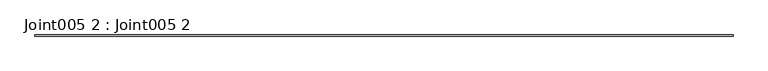
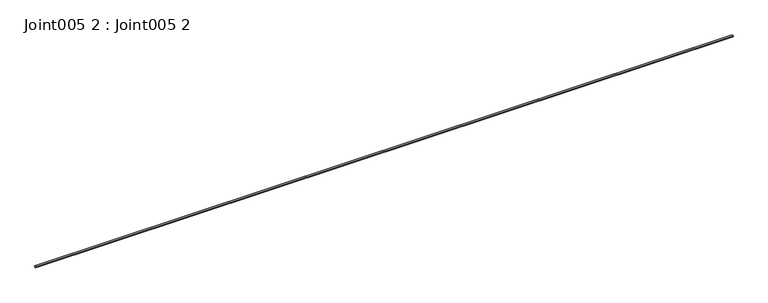
"""IFC4 building model written with IfcOpenShell, lengths in millimetres: proxy geometry, Joint005 2 : Joint005 2."""

from ifc_helpers import new_model, si_unit, point, frame, frame_2d, origin, place, context, project, spatial, polyline, circle_curve, trimmed, segment, composite_curve, outline, extrude, source, transform, mapped, element, save


def joint005_2_joint005_2_2fc430ad(model_context):
    return source(origin(), model_context, "Body", "SweptSolid", [
        extrude(outline(composite_curve([segment(polyline([(10407.9541245, 42894.7389688), (10407.9541245, 42890.821)]), True, "CONTINUOUS"), segment(trimmed(circle_curve(frame_2d((10406.3557924, 42885.649125)), 5.4132205), [point((10407.9541245, 42890.821))], [point((10404.7574604, 42890.821))], True, "CARTESIAN"), True, "CONTINUOUS"), segment(polyline([(10404.7574604, 42890.821), (10404.7574604, 42894.7389688)]), True, "CONTINUOUS"), segment(trimmed(circle_curve(frame_2d((10406.3557924, 42889.5670938)), 5.4132205), [point((10404.7574604, 42894.7389688))], [point((10407.9541245, 42894.7389688))], False, "CARTESIAN"), True, "CONTINUOUS")], self_intersect=False)), frame((3694.2883192, 0.0, 0.0), z_axis=(1.0, 0.0, 0.0), x_axis=(0.0, 1.0, 0.0)), (0.0, 0.0, 1.0), 2000.0),
    ])


if __name__ == "__main__":
    model = new_model("IFC4")
    model_context = context("Model", 3, world=origin())
    ifc_project = project(units=[si_unit("LENGTHUNIT", "METRE", prefix="MILLI")], contexts=[model_context])
    site = spatial("IfcSite", under=ifc_project)
    building = spatial("IfcBuilding", under=site)
    placement = place(None, origin())
    joint005_2_joint005_2_shape = joint005_2_joint005_2_2fc430ad(model_context)
    element("IfcBuildingElementProxy", 1, Name="Joint005 2 : Joint005 2", ObjectType="Joint005 2 : Joint005 2", at=placement, inside=building, context=model_context, shape_type="MappedRepresentation", body=[
        mapped(joint005_2_joint005_2_shape, transform((0.0, 0.0, 0.0), x_axis=(1.0, 0.0, 0.0), y_axis=(0.0, 1.0, 0.0), z_axis=(0.0, 0.0, 1.0))),
    ])
    save(model, "model.ifc")

# Revit data of these elements
# Type "Joint005 2 : Joint005 2"
#   NameOverride = "Joint005"
# Element 1 (IfcBuildingElementProxy, "Joint005 2 : Joint005 2")
#   Materials on its faces: "SEALANT JOINT"
# Materials
#   "SEALANT JOINT": class "Unassigned", colour RGB 142 225 148, transparency 0
